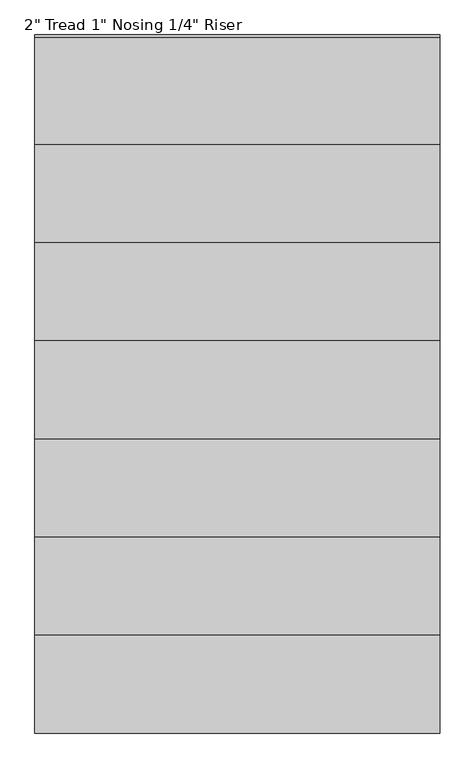
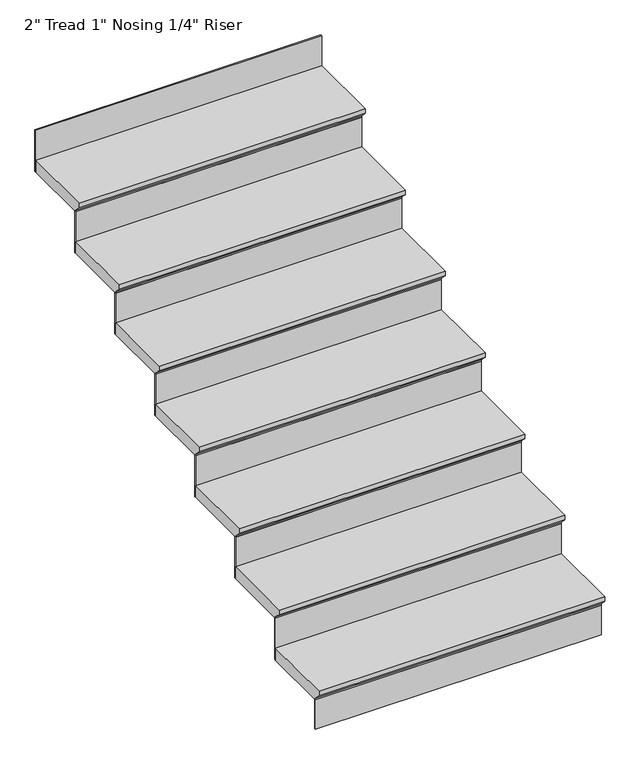
"""IFC4 building model written with IfcOpenShell, lengths in millimetres: stair flight geometry."""

from ifc_helpers import new_model, si_unit, frame, origin, origin_with_axes, place, context, project, spatial, polyline, outline, extrude, source, transform, mapped, element, save


def stair_flight_df08961e(model_context):
    return source(origin(), model_context, "Body", "SweptSolid", [
        extrude(outline(polyline([(15183.9212442, 177.8), (15488.7212442, 177.8), (15488.7212442, 127.0), (15209.3212442, 127.0), (15209.3212442, 133.35), (15183.9212442, 158.75), (15183.9212442, 177.8)])), frame((-328.6436975, 0.0, 0.0), z_axis=(1.0, 0.0, 0.0), x_axis=(0.0, 1.0, 0.0)), (0.0, 0.0, 1.0), 1154.2700538),
        extrude(outline(polyline([(825.6263562, 15215.6712442), (825.6263562, 15209.3212442), (-328.6436975, 15209.3212442), (-328.6436975, 15215.6712442), (825.6263562, 15215.6712442)])), origin_with_axes(), (0.0, 0.0, 1.0), 127.0),
        extrude(outline(polyline([(825.6263562, 15495.0712442), (825.6263562, 15488.7212442), (-328.6436975, 15488.7212442), (-328.6436975, 15495.0712442), (825.6263562, 15495.0712442)])), frame((0.0, 0.0, 127.0), z_axis=(0.0, 0.0, 1.0), x_axis=(1.0, 0.0, 0.0)), (0.0, 0.0, 1.0), 177.8),
        extrude(outline(polyline([(15463.3212442, 355.6), (15768.1212442, 355.6), (15768.1212442, 304.8), (15488.7212442, 304.8), (15488.7212442, 311.15), (15463.3212442, 336.55), (15463.3212442, 355.6)])), frame((-328.6436975, 0.0, 0.0), z_axis=(1.0, 0.0, 0.0), x_axis=(0.0, 1.0, 0.0)), (0.0, 0.0, 1.0), 1154.2700538),
        extrude(outline(polyline([(825.6263562, 15774.4712442), (825.6263562, 15768.1212442), (-328.6436975, 15768.1212442), (-328.6436975, 15774.4712442), (825.6263562, 15774.4712442)])), frame((0.0, 0.0, 304.8), z_axis=(0.0, 0.0, 1.0), x_axis=(1.0, 0.0, 0.0)), (0.0, 0.0, 1.0), 177.8),
        extrude(outline(polyline([(15742.7212442, 533.4), (16047.5212442, 533.4), (16047.5212442, 482.6), (15768.1212442, 482.6), (15768.1212442, 488.95), (15742.7212442, 514.35), (15742.7212442, 533.4)])), frame((-328.6436975, 0.0, 0.0), z_axis=(1.0, 0.0, 0.0), x_axis=(0.0, 1.0, 0.0)), (0.0, 0.0, 1.0), 1154.2700538),
        extrude(outline(polyline([(825.6263562, 16053.8712442), (825.6263562, 16047.5212442), (-328.6436975, 16047.5212442), (-328.6436975, 16053.8712442), (825.6263562, 16053.8712442)])), frame((0.0, 0.0, 482.6), z_axis=(0.0, 0.0, 1.0), x_axis=(1.0, 0.0, 0.0)), (0.0, 0.0, 1.0), 177.8),
        extrude(outline(polyline([(16022.1212442, 711.2), (16326.9212442, 711.2), (16326.9212442, 660.4), (16047.5212442, 660.4), (16047.5212442, 666.75), (16022.1212442, 692.15), (16022.1212442, 711.2)])), frame((-328.6436975, 0.0, 0.0), z_axis=(1.0, 0.0, 0.0), x_axis=(0.0, 1.0, 0.0)), (0.0, 0.0, 1.0), 1154.2700538),
        extrude(outline(polyline([(825.6263562, 16333.2712442), (825.6263562, 16326.9212442), (-328.6436975, 16326.9212442), (-328.6436975, 16333.2712442), (825.6263562, 16333.2712442)])), frame((0.0, 0.0, 660.4), z_axis=(0.0, 0.0, 1.0), x_axis=(1.0, 0.0, 0.0)), (0.0, 0.0, 1.0), 177.8),
        extrude(outline(polyline([(16301.5212442, 889.0), (16606.3212442, 889.0), (16606.3212442, 838.2), (16326.9212442, 838.2), (16326.9212442, 844.55), (16301.5212442, 869.95), (16301.5212442, 889.0)])), frame((-328.6436975, 0.0, 0.0), z_axis=(1.0, 0.0, 0.0), x_axis=(0.0, 1.0, 0.0)), (0.0, 0.0, 1.0), 1154.2700538),
        extrude(outline(polyline([(825.6263562, 16612.6712442), (825.6263562, 16606.3212442), (-328.6436975, 16606.3212442), (-328.6436975, 16612.6712442), (825.6263562, 16612.6712442)])), frame((0.0, 0.0, 838.2), z_axis=(0.0, 0.0, 1.0), x_axis=(1.0, 0.0, 0.0)), (0.0, 0.0, 1.0), 177.8),
        extrude(outline(polyline([(16580.9212442, 1066.8), (16885.7212442, 1066.8), (16885.7212442, 1016.0), (16606.3212442, 1016.0), (16606.3212442, 1022.35), (16580.9212442, 1047.75), (16580.9212442, 1066.8)])), frame((-328.6436975, 0.0, 0.0), z_axis=(1.0, 0.0, 0.0), x_axis=(0.0, 1.0, 0.0)), (0.0, 0.0, 1.0), 1154.2700538),
        extrude(outline(polyline([(825.6263562, 16892.0712442), (825.6263562, 16885.7212442), (-328.6436975, 16885.7212442), (-328.6436975, 16892.0712442), (825.6263562, 16892.0712442)])), frame((0.0, 0.0, 1016.0), z_axis=(0.0, 0.0, 1.0), x_axis=(1.0, 0.0, 0.0)), (0.0, 0.0, 1.0), 177.8),
        extrude(outline(polyline([(825.6263562, 17171.4712442), (825.6263562, 17165.1212442), (-328.6436975, 17165.1212442), (-328.6436975, 17171.4712442), (825.6263562, 17171.4712442)])), frame((0.0, 0.0, 1193.8), z_axis=(0.0, 0.0, 1.0), x_axis=(1.0, 0.0, 0.0)), (0.0, 0.0, 1.0), 177.8),
        extrude(outline(polyline([(16860.3212442, 1244.6), (17165.1212442, 1244.6), (17165.1212442, 1193.8), (16885.7212442, 1193.8), (16885.7212442, 1200.15), (16860.3212442, 1225.55), (16860.3212442, 1244.6)])), frame((-328.6436975, 0.0, 0.0), z_axis=(1.0, 0.0, 0.0), x_axis=(0.0, 1.0, 0.0)), (0.0, 0.0, 1.0), 1154.2700538),
    ])


if __name__ == "__main__":
    model = new_model("IFC4")
    model_context = context("Model", 3, world=origin())
    ifc_project = project(units=[si_unit("LENGTHUNIT", "METRE", prefix="MILLI")], contexts=[model_context])
    site = spatial("IfcSite", under=ifc_project)
    building = spatial("IfcBuilding", under=site)
    placement = place(None, origin())
    stair_flight_shape = stair_flight_df08961e(model_context)
    element("IfcStairFlight", 1, ObjectType="2\" Tread 1\" Nosing 1/4\" Riser", at=placement, inside=building, context=model_context, shape_type="MappedRepresentation", body=[
        mapped(stair_flight_shape, transform((0.0, 0.0, 0.0), x_axis=(1.0, 0.0, 0.0), y_axis=(0.0, 1.0, 0.0), z_axis=(0.0, 0.0, 1.0))),
    ])
    save(model, "model.ifc")

# Revit data of these elements
# Element 1 (IfcStairFlight, "2\" Tread 1\" Nosing 1/4\" Riser")
#   Materials on its faces: "Garpet - Sea Green"
# Materials
#   "Garpet - Sea Green": class "Carpet", colour RGB 107 175 109, transparency 0, Cost = 0
